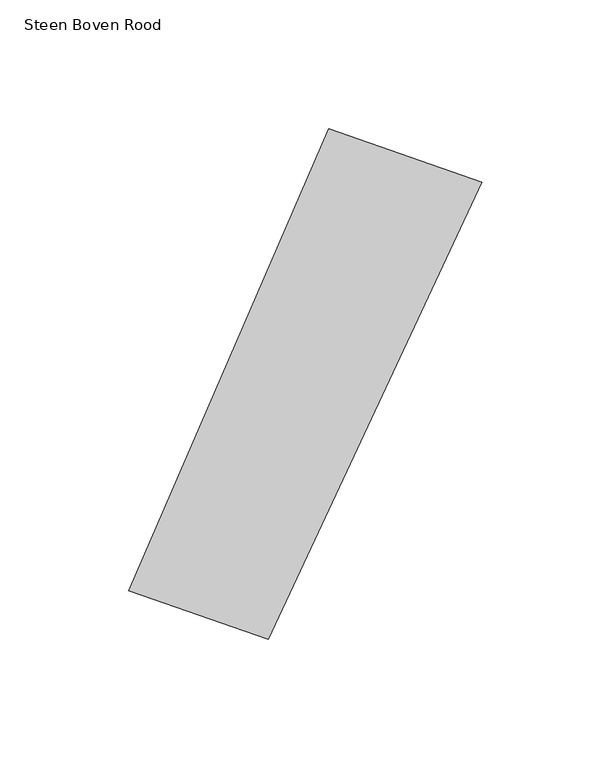
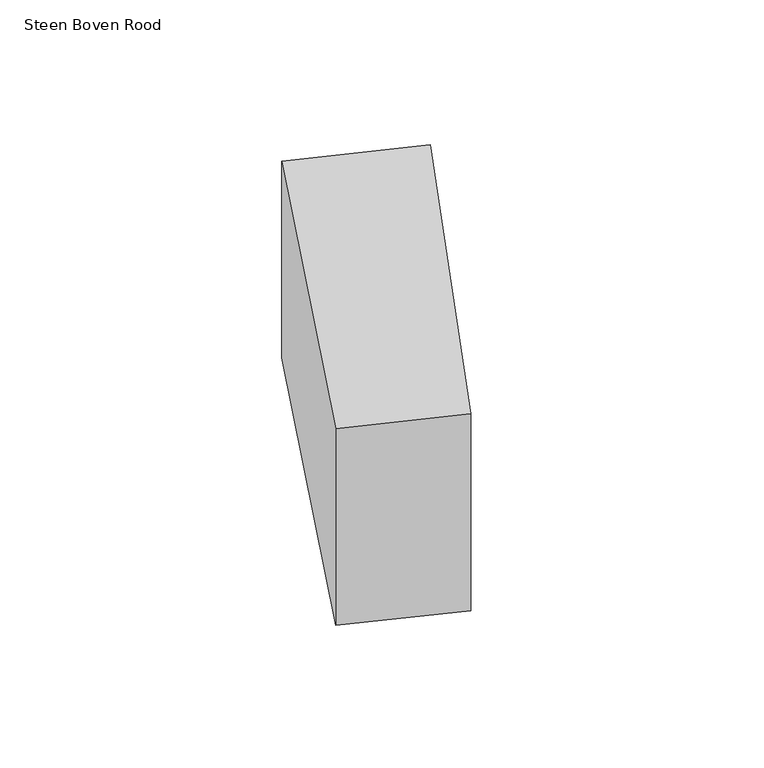
"""IFC4 building model written with IfcOpenShell, lengths in millimetres: proxy geometry, 00_GMA_steen_versie_4 : Steen Boven Rood."""

from ifc_helpers import new_model, si_unit, origin, origin_with_axes, place, context, project, spatial, polyline, outline, extrude, source, transform, mapped, element, save


def steen_boven_rood_75c40021(model_context):
    return source(origin(), model_context, "Body", "SweptSolid", [
        extrude(outline(polyline([(143.4107902, 161.300983), (60.3710173, -16.2863601), (6.1970973, 2.6108491), (83.8494144, 182.0649118), (143.4107902, 161.300983)])), origin_with_axes(), (0.0, 0.0, 1.0), 100.0),
    ])


if __name__ == "__main__":
    model = new_model("IFC4")
    model_context = context("Model", 3, world=origin())
    ifc_project = project(units=[si_unit("LENGTHUNIT", "METRE", prefix="MILLI")], contexts=[model_context])
    site = spatial("IfcSite", under=ifc_project)
    building = spatial("IfcBuilding", under=site)
    placement = place(None, origin())
    steen_boven_rood_shape = steen_boven_rood_75c40021(model_context)
    element("IfcBuildingElementProxy", 1, Name="00_GMA_steen_versie_4 : Steen Boven Rood", ObjectType="00_GMA_steen_versie_4 : Steen Boven Rood", at=placement, inside=building, context=model_context, shape_type="MappedRepresentation", body=[
        mapped(steen_boven_rood_shape, transform((0.0, 0.0, 0.0), x_axis=(1.0, 0.0, 0.0), y_axis=(0.0, 1.0, 0.0), z_axis=(0.0, 0.0, 1.0))),
    ])
    save(model, "model.ifc")

# Revit data of these elements
# Type "00_GMA_steen_versie_4 : Steen Boven Rood"
#   StootVoegHalfBoven [instance default] = 5 mm
#   StootVoegHalf [instance default] = 5 mm
#   StootVoegBreedteOnder = 10 mm
#   StootVoegBreedteBoven = 10 mm
#   Steendikte = 100 mm
#   LintVoegOnderHalf = 5 mm
#   LintVoegOnder = 10 mm
#   LintVoegBovenHalf = 0 mm
#   LintVoegBoven = 0 mm
#   materiaal = 21_steen_rood
#   MateriaalVoeg = none
#   Default Elevation = 0
# Element 1 (IfcBuildingElementProxy, "00_GMA_steen_versie_4 : Steen Boven Rood")
#   Materials on its faces: "21_steen_rood"
# Materials
#   "21_steen_rood": class "Unassigned", colour RGB 213 111 43, transparency 0, Cost = 0
